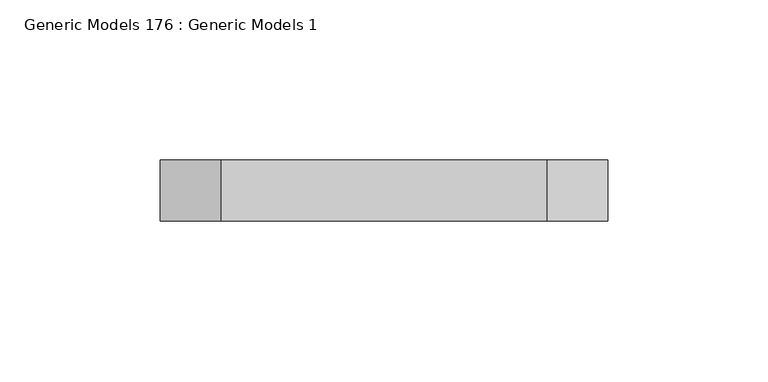
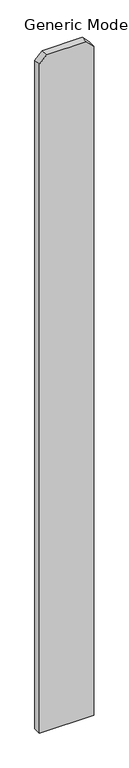
"""IFC4 building model written with IfcOpenShell, lengths in millimetres: proxy geometry, Generic Models 176 : Generic Models 1."""

import ifcopenshell
import ifcopenshell.guid

model = None  # the IFC model being written
_history = None  # IfcOwnerHistory: only IFC2X3 demands one
_inside = {}  # id of a spatial element -> (the spatial element, [elements in it])
_under = {}  # id of a project, library or spatial element -> (it, [spatial elements below it])
_declared = {}  # id of a project -> (the project, [libraries it declares])
_typed = {}  # id of a type object -> (the type object, [elements of that type])
_made_of = {}  # id of a material, layer set ... -> (it, [elements and type objects made of it])


def new_model(schema):
    """Start an empty IFC model of exactly this schema.

    Asked for "IFC4X3", IfcOpenShell would pick the latest addendum, in which some entities
    have other attributes; the version numbers below select the first issue.
    IFC2X3 requires an IfcOwnerHistory on every rooted entity: one is made here for all.
    """
    global model, _history
    if schema == "IFC4X3":
        model = ifcopenshell.file(schema_version=(4, 3, 0, 0))
    else:
        model = ifcopenshell.file(schema=schema)
    _inside.clear()
    _under.clear()
    _declared.clear()
    _typed.clear()
    _made_of.clear()
    _history = None
    if model.schema == "IFC2X3":
        org = make("IfcOrganization", Name="unknown")
        user = make(
            "IfcPersonAndOrganization",
            ThePerson=make("IfcPerson", FamilyName="unknown"),
            TheOrganization=org,
        )
        app = make(
            "IfcApplication",
            ApplicationDeveloper=org,
            Version="unknown",
            ApplicationFullName="unknown",
            ApplicationIdentifier="unknown",
        )
        _history = make(
            "IfcOwnerHistory",
            OwningUser=user,
            OwningApplication=app,
            ChangeAction="ADDED",
            CreationDate=0,
        )
    return model


def make(cls, **values):
    """One entity of the class cls with the attributes given. An attribute that is None is left unset."""
    return model.create_entity(
        cls, **{name: value for name, value in values.items() if value is not None}
    )


def rooted(cls, **values):
    """An entity with a GlobalId (a new one), such as an element, a storey or a relation."""
    return make(cls, GlobalId=ifcopenshell.guid.new(), OwnerHistory=_history, **values)


def si_unit(unit_type, name, prefix=None):
    """IfcSIUnit, for example si_unit("LENGTHUNIT", "METRE", prefix="MILLI")."""
    return make("IfcSIUnit", UnitType=unit_type, Prefix=prefix, Name=name)


def assignment(units):
    """IfcUnitAssignment: the units of a project."""
    return None if units is None else make("IfcUnitAssignment", Units=units)


def point(xyz):
    """IfcCartesianPoint."""
    return None if xyz is None else make("IfcCartesianPoint", Coordinates=xyz)


def direction(xyz):
    """IfcDirection."""
    return None if xyz is None else make("IfcDirection", DirectionRatios=xyz)


def frame(location, z_axis=None, x_axis=None):
    """IfcAxis2Placement3D, a coordinate frame: its origin and axes. An axis left out is left unset."""
    return make(
        "IfcAxis2Placement3D",
        Location=point(location),
        Axis=direction(z_axis),
        RefDirection=direction(x_axis),
    )


def origin():
    """The frame at (0, 0, 0) with its axes left unset."""
    return frame((0.0, 0.0, 0.0))


def place(relative_to, where):
    """IfcLocalPlacement: puts the frame where relative to a parent placement (None: the world)."""
    return make(
        "IfcLocalPlacement", PlacementRelTo=relative_to, RelativePlacement=where
    )


def context(
    kind, dimensions, precision=None, world=None, true_north=None, identifier=None
):
    """IfcGeometricRepresentationContext, for example the 3D "Model" context."""
    return make(
        "IfcGeometricRepresentationContext",
        ContextIdentifier=identifier,
        ContextType=kind,
        CoordinateSpaceDimension=dimensions,
        Precision=precision,
        WorldCoordinateSystem=world,
        TrueNorth=true_north,
    )


def project(units=None, contexts=None):
    """IfcProject with its units and contexts."""
    return rooted(
        "IfcProject",
        Name="project",
        RepresentationContexts=contexts,
        UnitsInContext=assignment(units),
    )


def spatial(cls, under=None, at=None, **own):
    """A site, building, storey or space (cls), placed at a placement, below another one or the project."""
    s = rooted(cls, ObjectPlacement=at, **own)
    if under is not None:
        _under.setdefault(under.id(), (under, []))[1].append(s)
    return s


def polyline(points):
    """IfcPolyline through the points."""
    return make("IfcPolyline", Points=[point(p) for p in points])


def outline(outer, holes=None, kind="AREA"):
    """IfcArbitraryClosedProfileDef: a profile drawn as a closed curve; with holes, ...WithVoids."""
    if holes is None:
        return make("IfcArbitraryClosedProfileDef", ProfileType=kind, OuterCurve=outer)
    return make(
        "IfcArbitraryProfileDefWithVoids",
        ProfileType=kind,
        OuterCurve=outer,
        InnerCurves=holes,
    )


def extrude(swept, where, along, depth):
    """IfcExtrudedAreaSolid: the profile swept, set in the frame where, extruded along a direction by depth."""
    return make(
        "IfcExtrudedAreaSolid",
        SweptArea=swept,
        Position=where,
        ExtrudedDirection=direction(along),
        Depth=depth,
    )


def shape(context_of_items, identifier, shape_type, items):
    """IfcShapeRepresentation: the items that make up one representation, for example the "Body"."""
    return make(
        "IfcShapeRepresentation",
        ContextOfItems=context_of_items,
        RepresentationIdentifier=identifier,
        RepresentationType=shape_type,
        Items=items,
    )


def source(mapping_origin, context_of_items, identifier, shape_type, items):
    """IfcRepresentationMap: a shape defined once, which mapped items show again and again."""
    return make(
        "IfcRepresentationMap",
        MappingOrigin=mapping_origin,
        MappedRepresentation=shape(context_of_items, identifier, shape_type, items),
    )


def transform(
    local_origin,
    x_axis=None,
    y_axis=None,
    z_axis=None,
    scale=None,
    scale2=None,
    scale3=None,
    uniform=True,
):
    """IfcCartesianTransformationOperator3D, or its non-uniform kind. x_axis, y_axis, z_axis: its Axis1, 2, 3."""
    if uniform:
        return make(
            "IfcCartesianTransformationOperator3D",
            Axis1=direction(x_axis),
            Axis2=direction(y_axis),
            LocalOrigin=point(local_origin),
            Scale=scale,
            Axis3=direction(z_axis),
        )
    return make(
        "IfcCartesianTransformationOperator3DnonUniform",
        Axis1=direction(x_axis),
        Axis2=direction(y_axis),
        LocalOrigin=point(local_origin),
        Scale=scale,
        Axis3=direction(z_axis),
        Scale2=scale2,
        Scale3=scale3,
    )


def mapped(mapping_source, mapping_target):
    """IfcMappedItem: shows the shape of a source again, moved by a transform."""
    return make(
        "IfcMappedItem", MappingSource=mapping_source, MappingTarget=mapping_target
    )


def made_of(thing, what):
    """Note that an element or type object is made of a material, layer set ...; save() writes the relation."""
    if what is not None:
        _made_of.setdefault(what.id(), (what, []))[1].append(thing)
    return thing


def element(
    cls,
    number,
    at=None,
    inside=None,
    cuts=None,
    type_object=None,
    material=None,
    context=None,
    identifier="Body",
    shape_type=None,
    held_by="IfcProductDefinitionShape",
    body=None,
    shapes=None,
    **own,
):
    """One element of the class cls, such as IfcWall. Its Tag is "e" and its number.

    at: its placement. inside: the storey or other place that contains it. cuts: it is an
    opening in that element (IfcRelVoidsElement). A single representation is given by context,
    identifier, shape_type and body (its items); several are given by shapes. held_by: the class
    of the entity that holds the representations. save() writes the other relations.
    """
    e = rooted(cls, Tag="e%d" % number, ObjectPlacement=at, **own)
    if body is not None:
        shapes = [shape(context, identifier, shape_type, body)]
    if shapes is not None:
        e.Representation = make(held_by, Representations=shapes)
    if inside is not None:
        _inside.setdefault(inside.id(), (inside, []))[1].append(e)
    if cuts is not None:
        rooted(
            "IfcRelVoidsElement", RelatingBuildingElement=cuts, RelatedOpeningElement=e
        )
    if type_object is not None:
        _typed.setdefault(type_object.id(), (type_object, []))[1].append(e)
    return made_of(e, material)


def aggregate(whole, parts):
    """IfcRelAggregates: a whole, such as a stair, and the parts it consists of."""
    return rooted("IfcRelAggregates", RelatingObject=whole, RelatedObjects=parts)


def save(model, path):
    """Write the relations noted so far, then the file.

    IfcRelAggregates (storeys below a building ...), IfcRelContainedInSpatialStructure (elements
    in a storey), IfcRelDefinesByType, IfcRelAssociatesMaterial and IfcRelDeclares: one each for
    every whole, place, type object, material and project.
    """
    for whole, parts in _under.values():
        aggregate(whole, parts)
    for where, things in _inside.values():
        rooted(
            "IfcRelContainedInSpatialStructure",
            RelatedElements=things,
            RelatingStructure=where,
        )
    for kind, things in _typed.values():
        rooted("IfcRelDefinesByType", RelatedObjects=things, RelatingType=kind)
    for what, things in _made_of.values():
        rooted("IfcRelAssociatesMaterial", RelatedObjects=things, RelatingMaterial=what)
    for by, libraries in _declared.values():
        rooted("IfcRelDeclares", RelatingContext=by, RelatedDefinitions=libraries)
    model.write(path)


def generic_models_176_generic_models_1_de16f722(model_context):
    return source(origin(), model_context, "Body", "SweptSolid", [
        extrude(outline(polyline([(76.2, 56818.2125), (1885.95, 56818.2125), (1905.0, 56799.1625), (1905.0, 56697.5625), (1885.95, 56678.5125), (76.2, 56678.5125), (76.2, 56818.2125)])), frame((0.0, 547.6875, 0.0), z_axis=(0.0, 1.0, 0.0), x_axis=(0.0, 0.0, 1.0)), (0.0, 0.0, 1.0), 19.05),
    ])


if __name__ == "__main__":
    model = new_model("IFC4")
    model_context = context("Model", 3, world=origin())
    ifc_project = project(units=[si_unit("LENGTHUNIT", "METRE", prefix="MILLI")], contexts=[model_context])
    site = spatial("IfcSite", under=ifc_project)
    building = spatial("IfcBuilding", under=site)
    placement = place(None, origin())
    generic_models_176_generic_models_1_shape = generic_models_176_generic_models_1_de16f722(model_context)
    element("IfcBuildingElementProxy", 1, Name="Generic Models 176 : Generic Models 1", ObjectType="Generic Models 176 : Generic Models 1", at=placement, inside=building, context=model_context, shape_type="MappedRepresentation", body=[
        mapped(generic_models_176_generic_models_1_shape, transform((0.0, 0.0, 0.0), x_axis=(1.0, 0.0, 0.0), y_axis=(0.0, 1.0, 0.0), z_axis=(0.0, 0.0, 1.0))),
    ])
    save(model, "model.ifc")

# Revit data of these elements
# Element 1 (IfcBuildingElementProxy, "Generic Models 176 : Generic Models 1")
#   Materials on its faces: "VERTICAL 1X6 CEDAR PLANKS W/ CLEAR WOOD SEALER"
# Materials
#   "VERTICAL 1X6 CEDAR PLANKS W/ CLEAR WOOD SEALER": class "Wood", colour RGB 234 198 147, transparency 0, Description = "Pinus Echinata", Cost = 0
